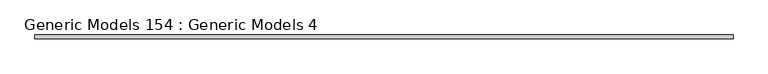
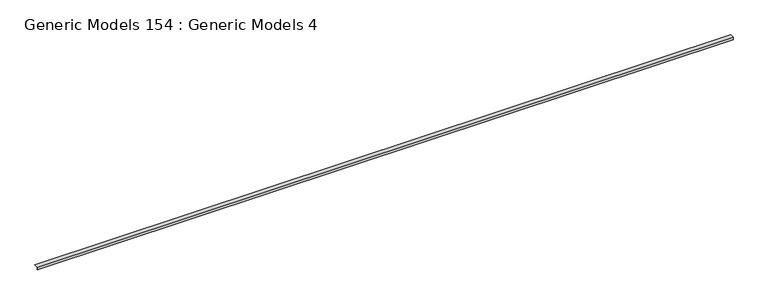
"""IFC4 building model written with IfcOpenShell, lengths in millimetres: proxy geometry, Generic Models 154 : Generic Models 4."""

from ifc_helpers import new_model, si_unit, frame, origin, place, context, project, spatial, polyline, outline, extrude, source, transform, mapped, element, save


def generic_models_154_generic_models_4_447907b8(model_context):
    return source(origin(), model_context, "Body", "SweptSolid", [
        extrude(outline(polyline([(6874.9428374, 124210.0975133), (6874.9428374, 124128.3114066), (6874.1490874, 124128.3114066), (6874.1490874, 124210.8912633), (6974.3071081, 124210.8912633), (6974.3071081, 124210.0975133), (6874.9428374, 124210.0975133)])), frame((-10234.5171316, 0.0, 0.0), z_axis=(1.0, 0.0, 0.0), x_axis=(0.0, 1.0, 0.0)), (0.0, 0.0, 1.0), 18643.6),
    ])


if __name__ == "__main__":
    model = new_model("IFC4")
    model_context = context("Model", 3, world=origin())
    ifc_project = project(units=[si_unit("LENGTHUNIT", "METRE", prefix="MILLI")], contexts=[model_context])
    site = spatial("IfcSite", under=ifc_project)
    building = spatial("IfcBuilding", under=site)
    placement = place(None, origin())
    generic_models_154_generic_models_4_shape = generic_models_154_generic_models_4_447907b8(model_context)
    element("IfcBuildingElementProxy", 1, Name="Generic Models 154 : Generic Models 4", ObjectType="Generic Models 154 : Generic Models 4", at=placement, inside=building, context=model_context, shape_type="MappedRepresentation", body=[
        mapped(generic_models_154_generic_models_4_shape, transform((0.0, 0.0, 0.0), x_axis=(1.0, 0.0, 0.0), y_axis=(0.0, 1.0, 0.0), z_axis=(0.0, 0.0, 1.0))),
    ])
    save(model, "model.ifc")

# Revit data of these elements
# Element 1 (IfcBuildingElementProxy, "Generic Models 154 : Generic Models 4")
#   Materials on its faces: "_SELF ADHERED MEMBRANE W/ END DAMS WHERE POSSIBLE"
# Materials
#   "_SELF ADHERED MEMBRANE W/ END DAMS WHERE POSSIBLE": class "Generic", colour RGB 253 192 103, transparency 0, Cost = 0
